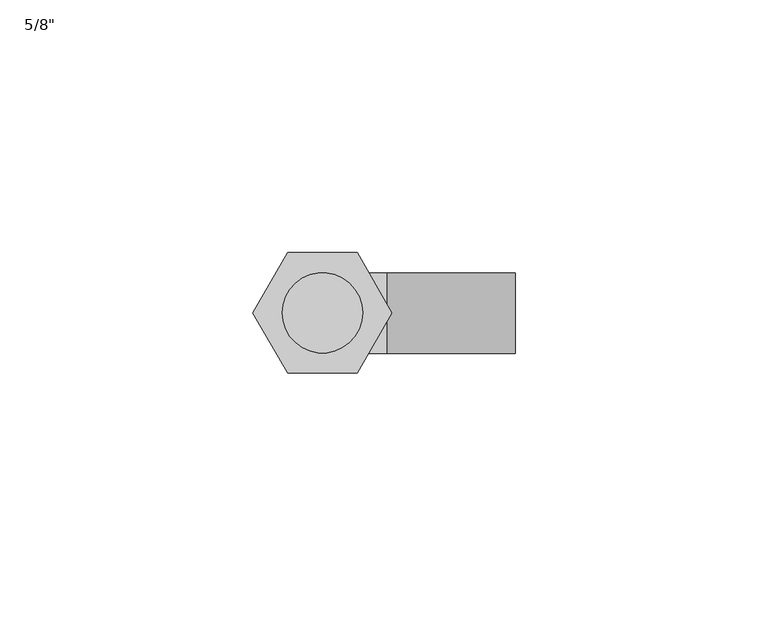
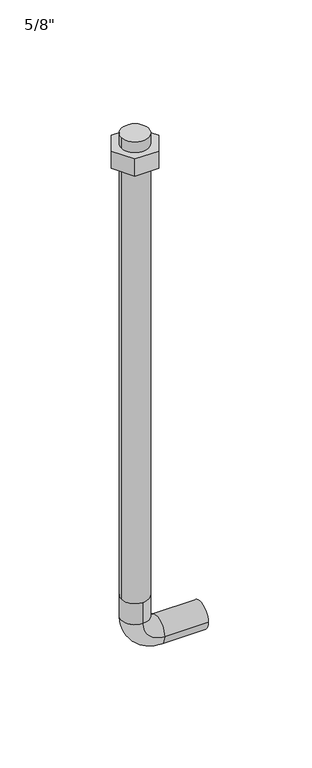
"""IFC4 building model written with IfcOpenShell, lengths in millimetres: proxy geometry."""

from ifc_helpers import new_model, si_unit, point, frame, origin, origin_with_axes, place, context, project, spatial, polyline, circle_curve, ellipse_curve, trimmed, outline, extrude, source, transform, mapped, element, save
from ifc_brep_helpers import plane_surface, cylinder_surface, revolved_surface, advanced_brep


def proxy_05963efa(model_context):
    return source(origin(), model_context, "Body", "SolidModel", [
        advanced_brep(
        [(0.0, -7.9375, -266.7), (-7.9375, 0.0, -266.7), (0.0, 7.9375, -266.7), (0.0, 7.9375, -279.4), (0.0, -7.9375, -279.4), (7.9375, 0.0, -266.7), (12.7, 7.9375, -292.1), (12.7, -7.9375, -292.1), (38.1, -7.9375, -292.1), (38.1, 7.9375, -292.1), (-7.9375, 0.0, 17.065625), (7.9375, 0.0, 17.065625)],
        [
            (0, 1, circle_curve(frame((0.0, 0.0, -266.7), z_axis=(0.0, 0.0, -1.0), x_axis=(0.0, 1.0, 0.0)), 7.9375)),
            (1, 2, circle_curve(frame((0.0, 0.0, -266.7), z_axis=(0.0, 0.0, -1.0), x_axis=(0.0, 1.0, 0.0)), 7.9375)),
            (2, 3),
            (3, 4, circle_curve(frame((0.0, 0.0, -279.4), z_axis=(0.0, 0.0, 1.0), x_axis=(0.0, 1.0, 0.0)), 7.9375)),
            (4, 0),
            (4, 3, circle_curve(frame((0.0, 0.0, -279.4), z_axis=(0.0, 0.0, 1.0), x_axis=(0.0, 1.0, 0.0)), 7.9375)),
            (2, 5, circle_curve(frame((0.0, 0.0, -266.7), z_axis=(0.0, 0.0, -1.0), x_axis=(0.0, 1.0, 0.0)), 7.9375)),
            (5, 0, circle_curve(frame((0.0, 0.0, -266.7), z_axis=(0.0, 0.0, -1.0), x_axis=(0.0, 1.0, 0.0)), 7.9375)),
            (3, 6, circle_curve(frame((12.7, 7.9375, -279.4), z_axis=(0.0, -1.0, 0.0), x_axis=(-1.0, 0.0, 0.0)), 12.7)),
            (6, 7, circle_curve(frame((12.7, 0.0, -292.1), z_axis=(-1.0, 0.0, 0.0), x_axis=(0.0, 1.0, 0.0)), 7.9375)),
            (7, 4, circle_curve(frame((12.7, -7.9375, -279.4), z_axis=(0.0, 1.0, 0.0), x_axis=(-1.0, 0.0, 0.0)), 12.7)),
            (7, 6, circle_curve(frame((12.7, 0.0, -292.1), z_axis=(-1.0, 0.0, 0.0), x_axis=(0.0, 1.0, 0.0)), 7.9375)),
            (8, 9, circle_curve(frame((38.1, 0.0, -292.1), z_axis=(1.0, 0.0, 0.0), x_axis=(0.0, 1.0, 0.0)), 7.9375)),
            (9, 8, circle_curve(frame((38.1, 0.0, -292.1), z_axis=(1.0, 0.0, 0.0), x_axis=(0.0, 1.0, 0.0)), 7.9375)),
            (6, 9),
            (8, 7),
            (10, 11, circle_curve(frame((0.0, 0.0, 17.065625), z_axis=(0.0, 0.0, 1.0), x_axis=(1.0, 0.0, 0.0)), 7.9375)),
            (11, 10, circle_curve(frame((0.0, 0.0, 17.065625), z_axis=(0.0, 0.0, 1.0), x_axis=(1.0, 0.0, 0.0)), 7.9375)),
            (11, 5),
            (1, 10),
        ],
        [
            cylinder_surface(frame((0.0, 0.0, -266.7), z_axis=(0.0, 0.0, 1.0), x_axis=(0.0, 1.0, 0.0)), 7.9375),
            revolved_surface(trimmed(ellipse_curve(frame((0.0, 0.0, -279.4), z_axis=(0.0, 0.0, -1.0), x_axis=(0.0, 1.0, 0.0)), 7.9375, 7.9375), [point((0.0, -7.9375, -279.4))], [point((0.0, 7.9375, -279.4))], True, "CARTESIAN"), (12.7, 0.0, -279.4), (0.0, 1.0, 0.0)),
            revolved_surface(trimmed(ellipse_curve(frame((0.0, 0.0, -279.4), z_axis=(0.0, 0.0, -1.0), x_axis=(0.0, 1.0, 0.0)), 7.9375, 7.9375), [point((0.0, 7.9375, -279.4))], [point((0.0, -7.9375, -279.4))], True, "CARTESIAN"), (12.7, 0.0, -279.4), (0.0, 1.0, 0.0)),
            plane_surface(frame((38.1, 0.0, -292.1), z_axis=(1.0, 0.0, 0.0), x_axis=(0.0, 1.0, 0.0))),
            cylinder_surface(frame((12.7, 0.0, -292.1), z_axis=(-1.0, 0.0, 0.0), x_axis=(0.0, 1.0, 0.0)), 7.9375),
            plane_surface(frame((7.9375, 0.0, 17.065625), z_axis=(0.0, 0.0, 1.0), x_axis=(0.0, -1.0, 0.0))),
            cylinder_surface(frame((0.0, 0.0, -266.7), z_axis=(0.0, 0.0, 1.0), x_axis=(1.0, 0.0, 0.0)), 7.9375),
        ],
        [
            (0, [[1, 2, 3, 4, 5]]),
            (0, [[6, -3, 7, 8, -5]]),
            (1, [[9, 10, 11, -4]]),
            (2, [[-11, 12, -9, -6]]),
            (3, [[13, 14]]),
            (4, [[15, -13, 16, -10]]),
            (4, [[-16, -14, -15, -12]]),
            (5, [[17, 18]]),
            (6, [[19, -7, -2, 20, -18]]),
            (6, [[-20, -1, -8, -19, -17]]),
        ],
    ),
        extrude(outline(polyline([(-13.7481533, 0.0), (-6.8740766, 11.90625), (6.8740766, 11.90625), (13.7481533, 0.0), (6.8740766, -11.90625), (-6.8740766, -11.90625), (-13.7481533, 0.0)])), origin_with_axes(), (0.0, 0.0, 1.0), 10.715625),
    ])


if __name__ == "__main__":
    model = new_model("IFC4")
    model_context = context("Model", 3, world=origin())
    ifc_project = project(units=[si_unit("LENGTHUNIT", "METRE", prefix="MILLI")], contexts=[model_context])
    site = spatial("IfcSite", under=ifc_project)
    building = spatial("IfcBuilding", under=site)
    placement = place(None, origin())
    proxy_shape = proxy_05963efa(model_context)
    element("IfcBuildingElementProxy", 1, Name="050523 - W_P_C - Fastenings - Bent Anchor Bolt : 5/8\"", ObjectType="050523 - W_P_C - Fastenings - Bent Anchor Bolt : 5/8\"", at=placement, inside=building, context=model_context, shape_type="MappedRepresentation", body=[
        mapped(proxy_shape, transform((0.0, 0.0, 0.0), x_axis=(1.0, 0.0, 0.0), y_axis=(0.0, 1.0, 0.0), z_axis=(0.0, 0.0, 1.0))),
    ])
    save(model, "model.ifc")

# Revit data of these elements
# Type "050523 - W_P_C - Fastenings - Bent Anchor Bolt : 5/8\""
#   Side = 0' - 0.54199"
#   Radius = 0' - 0 5/16"
#   Length = 0' - 10 1/2"
#   Head Size = 0' - 0 15/16"
#   Head Radius = 0' - 0 15/32"
#   Head Height = 0' - 0 27/64"
#   Diameter = 0' - 0 5/8"
#   Default Elevation = 4' - 0"
#   Bolt Material (Size) = 5/8” GALV. BENT ANCHOR BOLT @ 4’ O.C. (WITHIN 8” OF EVERY CORNER) 7” MIN. EMBEDMENT
# Element 1 (IfcBuildingElementProxy, "050523 - W_P_C - Fastenings - Bent Anchor Bolt : 5/8\"")
#   Materials on its faces: "5/8” GALV. BENT ANCHOR BOLT @ 4’ O.C. (WITHIN 8” OF EVERY CORNER) 7” MIN. EMBEDMENT"
# Materials
#   "5/8” GALV. BENT ANCHOR BOLT @ 4’ O.C. (WITHIN 8” OF EVERY CORNER) 7” MIN. EMBEDMENT": class "Generic", colour RGB 120 120 120, transparency 0, Cost = 0
